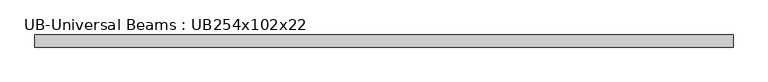
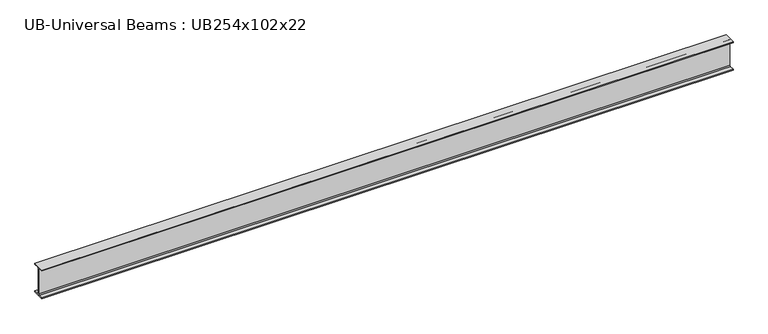
"""IFC4 building model written with IfcOpenShell, lengths in millimetres: beam geometry, UB-Universal Beams : UB254x102x22."""

from ifc_helpers import new_model, si_unit, point, frame, frame_2d, origin, place, context, project, spatial, polyline, circle_curve, trimmed, segment, composite_curve, outline, extrude, source, transform, mapped, element, save


def ub_universal_beams_ub254x102x22_c294fd8a(model_context):
    return source(origin(), model_context, "Body", "SweptSolid", [
        extrude(outline(composite_curve([segment(polyline([(50.8, -120.2), (50.8, -127.0), (-50.8, -127.0), (-50.8, -120.2), (-10.45, -120.2)]), True, "CONTINUOUS"), segment(trimmed(circle_curve(frame_2d((-10.45, -112.6)), 7.6), [point((-10.45, -120.2))], [point((-2.85, -112.6))], True, "CARTESIAN"), True, "CONTINUOUS"), segment(polyline([(-2.85, -112.6), (-2.85, 112.6)]), True, "CONTINUOUS"), segment(trimmed(circle_curve(frame_2d((-10.45, 112.6)), 7.6), [point((-2.85, 112.6))], [point((-10.45, 120.2))], True, "CARTESIAN"), True, "CONTINUOUS"), segment(polyline([(-10.45, 120.2), (-50.8, 120.2), (-50.8, 127.0), (50.8, 127.0), (50.8, 120.2), (10.45, 120.2)]), True, "CONTINUOUS"), segment(trimmed(circle_curve(frame_2d((10.45, 112.6)), 7.6), [point((10.45, 120.2))], [point((2.85, 112.6))], True, "CARTESIAN"), True, "CONTINUOUS"), segment(polyline([(2.85, 112.6), (2.85, -112.6)]), True, "CONTINUOUS"), segment(trimmed(circle_curve(frame_2d((10.45, -112.6)), 7.6), [point((2.85, -112.6))], [point((10.45, -120.2))], True, "CARTESIAN"), True, "CONTINUOUS"), segment(polyline([(10.45, -120.2), (50.8, -120.2)]), True, "CONTINUOUS")], self_intersect=False)), frame((-2936.5, 0.0, 0.0), z_axis=(1.0, 0.0, 0.0), x_axis=(0.0, 1.0, 0.0)), (0.0, 0.0, 1.0), 5847.6),
    ])


if __name__ == "__main__":
    model = new_model("IFC4")
    model_context = context("Model", 3, world=origin())
    ifc_project = project(units=[si_unit("LENGTHUNIT", "METRE", prefix="MILLI")], contexts=[model_context])
    site = spatial("IfcSite", under=ifc_project)
    building = spatial("IfcBuilding", under=site)
    placement = place(None, origin())
    ub_universal_beams_ub254x102x22_shape = ub_universal_beams_ub254x102x22_c294fd8a(model_context)
    element("IfcBeam", 1, ObjectType="UB-Universal Beams : UB254x102x22", at=placement, inside=building, context=model_context, shape_type="MappedRepresentation", body=[
        mapped(ub_universal_beams_ub254x102x22_shape, transform((0.0, 0.0, 0.0), x_axis=(1.0, 0.0, 0.0), y_axis=(0.0, 1.0, 0.0), z_axis=(0.0, 0.0, 1.0))),
    ])
    save(model, "model.ifc")

# Revit data of these elements
# Type "UB-Universal Beams : UB254x102x22"
#   Section Name Key = "UB254X102X22"
#   Width = 10.16 cm
#   Web Thickness = 0.57 cm
#   Web Fillet = 0.76 cm
#   Warping Constant = 18200.0 cm⁶
#   Torsional Moment of Inertia = 4.15 cm⁴
#   Section Area = 28.0 cm²
#   Plastic Modulus weak axis = 37.3 cm³
#   Plastic Modulus strong axis = 259.0 cm³
#   Nominal Weight = 22.00 kgf/m
#   Moment of Inertia weak axis = 119.00 cm⁴
#   Moment of Inertia strong axis = 2841.00 cm⁴
#   Height = 25.4 cm
#   Flange Thickness = 0.68 cm
#   Elastic Modulus weak axis = 23.5 cm³
#   Elastic Modulus strong axis = 224.0 cm³
#   Centroid Vertical = 12.7 cm
#   Centroid Horizontal = 5.08 cm
#   Bolt Spacing = 5.4 cm
#   Length [instance default] = 1500 mm
#   Structural Material [instance default] = Metal - Steel 43-275
#   Type Comments = ""
#   Assembly Code = ""
# Element 1 (IfcBeam, "UB-Universal Beams : UB254x102x22")
#   Materials on its faces: "Metal - Steel 43-275"
# Materials
#   "Metal - Steel 43-275": class "Metal", colour RGB 247 247 247, transparency 0, Cost = 0
